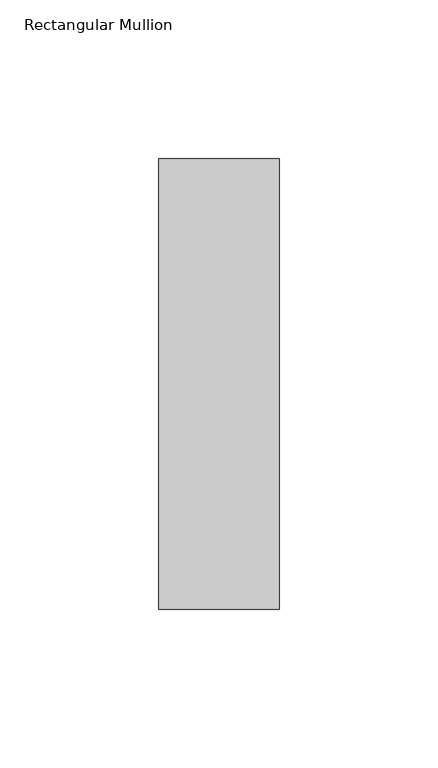
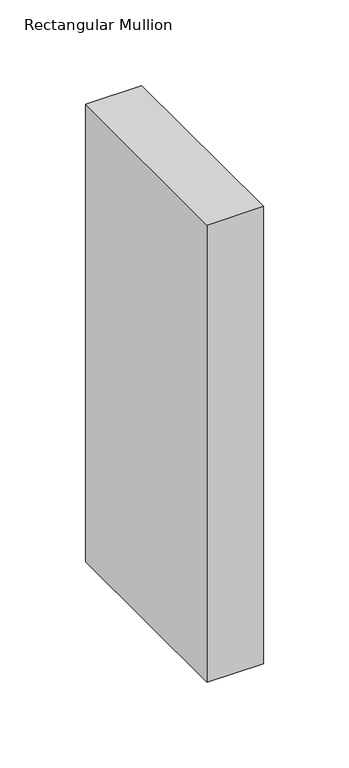
"""IFC4 building model written with IfcOpenShell, lengths in millimetres: member geometry, Rectangular Mullion : NLRS_21_CWM_hsb-regel 38x142_gen_rsf."""

from ifc_helpers import new_model, si_unit, frame, origin, place, context, project, spatial, polyline, outline, extrude, source, transform, mapped, element, save


def rectangular_mullion_610e01e3(model_context):
    return source(origin(), model_context, "Body", "SweptSolid", [
        extrude(outline(polyline([(0.0, -71.0), (-38.0, -71.0), (-38.0, 71.0), (0.0, 71.0), (0.0, -71.0)])), frame((0.0, 0.0, -326.0000003), z_axis=(0.0, 0.0, 1.0), x_axis=(1.0, 0.0, 0.0)), (0.0, 0.0, 1.0), 326.0000003),
    ])


if __name__ == "__main__":
    model = new_model("IFC4")
    model_context = context("Model", 3, world=origin())
    ifc_project = project(units=[si_unit("LENGTHUNIT", "METRE", prefix="MILLI")], contexts=[model_context])
    site = spatial("IfcSite", under=ifc_project)
    building = spatial("IfcBuilding", under=site)
    placement = place(None, origin())
    rectangular_mullion_shape = rectangular_mullion_610e01e3(model_context)
    element("IfcMember", 1, ObjectType="Rectangular Mullion : NLRS_21_CWM_hsb-regel 38x142_gen_rsf", at=placement, inside=building, context=model_context, shape_type="MappedRepresentation", body=[
        mapped(rectangular_mullion_shape, transform((0.0, 0.0, 0.0), x_axis=(1.0, 0.0, 0.0), y_axis=(0.0, 1.0, 0.0), z_axis=(0.0, 0.0, 1.0))),
    ])
    save(model, "model.ifc")

# Revit data of these elements
# Type "Rectangular Mullion : NLRS_21_CWM_hsb-regel 38x142_gen_rsf"
#   Export Type to IFC As = "IfcWall"
#   Type IfcGUID = "07M7mRoiH1CR8m_RSKIwpF"
#   Assembly Code = "21.10"
#   built-in parameter 1007322 = 0.465879 (stored number, unit not read)
#   built-in parameter 1007321 = 0.062336 (stored number, unit not read)
#   built-in parameter 1007320 = 0.062336 (stored number, unit not read)
# Element 1 (IfcMember, "Rectangular Mullion : NLRS_21_CWM_hsb-regel 38x142_gen_rsf")
#   Materials on its faces: "NLRS_i2_hout naaldhout vuren_gen_rsf"
# Materials
#   "NLRS_i2_hout naaldhout vuren_gen_rsf": class "I - Hout", colour RGB 234 199 147, transparency 0, Keynote = "i2", Manufacturer = "Revit Standards Foundation", URL = "www.revitstandards.org", Description = "hout vuren", Cost = 0
